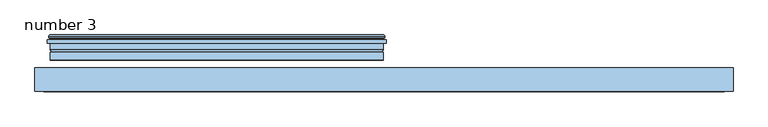
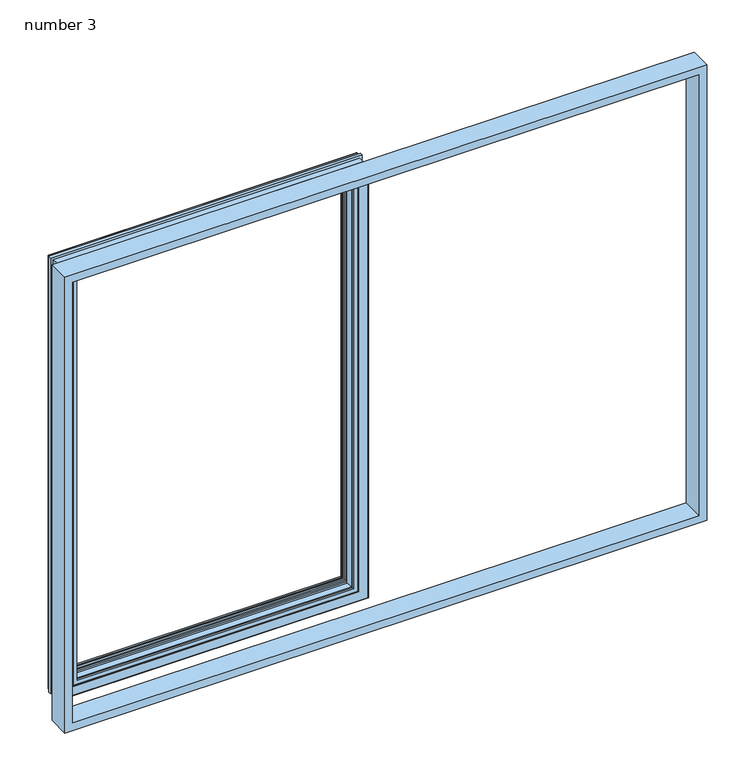
"""IFC4 building model written with IfcOpenShell, lengths in millimetres: window geometry, Window-Exterior-Sierra-Horizontal_Sliding_XO-36inch_Width-Standard : number 3."""

from ifc_helpers import new_model, si_unit, frame, origin, place, context, project, spatial, polyline, ellipse_curve, outline, extrude, source, transform, mapped, element, save
from ifc_brep_helpers import plane_surface, cylinder_surface, revolved_surface, advanced_brep


def number_3_e313addd(model_context):
    return source(origin(), model_context, "Body", "SolidModel", [
        advanced_brep(
        [(-554.92015, 35.099625, 967.49235), (-554.92015, 33.9637671, 967.49235), (-29.27985, 33.9637671, 967.49235), (-29.27985, 35.099625, 967.49235), (-553.0833265, 37.5426644, 969.3291735), (-552.8937762, 35.099625, 969.5187238), (-31.3062238, 35.099625, 969.5187238), (-31.1166735, 37.5426644, 969.3291735), (-560.88915, 40.078025, 961.52335), (-23.31085, 40.078025, 961.52335), (-560.88915, 42.465625, 961.52335), (-23.31085, 42.465625, 961.52335), (-585.57795, 40.078025, 936.83455), (-583.19035, 42.465625, 939.22215), (-1.00965, 42.465625, 939.22215), (1.37795, 40.078025, 936.83455), (-585.57795, 37.512625, 936.83455), (1.37795, 37.512625, 936.83455), (-583.54595, 35.836225, 938.86655), (-583.54595, 37.512625, 938.86655), (-0.65405, 37.512625, 938.86655), (-0.65405, 35.836225, 938.86655), (-580.24395, 33.931225, 942.16855), (-580.24395, 35.836225, 942.16855), (-3.95605, 35.836225, 942.16855), (-3.95605, 33.931225, 942.16855), (-588.16875, 28.317825, 934.24375), (-588.16875, 33.931225, 934.24375), (3.96875, 33.931225, 934.24375), (3.96875, 28.317825, 934.24375), (-582.86015, 16.125825, 939.55235), (-582.86015, 28.317825, 939.55235), (-1.33985, 28.317825, 939.55235), (-1.33985, 16.125825, 939.55235), (-582.86015, 12.163425, 939.55235), (-1.33985, 12.163425, 939.55235), (-582.86015, -1.171575, 939.55235), (-1.33985, -1.171575, 939.55235), (-582.04735, -1.984375, 940.36515), (-2.15265, -1.984375, 940.36515), (-563.75935, -0.103857, 958.65315), (-563.75935, -1.984375, 958.65315), (-20.44065, -1.984375, 958.65315), (-20.44065, -0.103857, 958.65315), (-562.1584612, -1.704057, 960.2540388), (-562.1584612, -0.103857, 960.2540388), (-22.0415388, -0.103857, 960.2540388), (-22.0415388, -1.704057, 960.2540388), (-554.6146612, 2.0638625, 967.7978388), (-554.6146612, -1.704057, 967.7978388), (-29.5853388, -1.704057, 967.7978388), (-29.5853388, 2.0638625, 967.7978388), (-551.4396612, 13.891543, 970.9728388), (-552.4523112, 2.0638625, 969.9601888), (-31.7476888, 2.0638625, 969.9601888), (-32.7603388, 13.891543, 970.9728388), (-563.75935, 11.5032541, 958.65315), (-561.3710612, 13.891543, 961.0414388), (-22.8289388, 13.891543, 961.0414388), (-20.44065, 11.5032541, 958.65315), (-563.75935, 32.940625, 958.65315), (-20.44065, 32.940625, 958.65315), (-559.1555891, 33.9637671, 963.2569109), (-560.1787312, 32.940625, 962.2337688), (-24.0212688, 32.940625, 962.2337688), (-25.0444109, 33.9637671, 963.2569109), (-29.27985, 33.9637671, 1775.70765), (-29.27985, 35.099625, 1775.70765), (-31.3062238, 35.099625, 1773.6812762), (-31.1166735, 37.5426644, 1773.8708265), (-23.31085, 40.078025, 1781.67665), (-23.31085, 42.465625, 1781.67665), (-1.00965, 42.465625, 1803.97785), (1.37795, 40.078025, 1806.36545), (1.37795, 37.512625, 1806.36545), (-0.65405, 37.512625, 1804.33345), (-0.65405, 35.836225, 1804.33345), (-3.95605, 35.836225, 1801.03145), (-3.95605, 33.931225, 1801.03145), (3.96875, 33.931225, 1808.95625), (3.96875, 28.317825, 1808.95625), (-1.33985, 28.317825, 1803.64765), (-1.33985, 16.125825, 1803.64765), (-1.33985, 12.163425, 1803.64765), (-1.33985, -1.171575, 1803.64765), (-2.15265, -1.984375, 1802.83485), (-20.44065, -1.984375, 1784.54685), (-20.44065, -0.103857, 1784.54685), (-22.0415388, -0.103857, 1782.9459612), (-22.0415388, -1.704057, 1782.9459612), (-29.5853388, -1.704057, 1775.4021612), (-29.5853388, 2.0638625, 1775.4021612), (-31.7476888, 2.0638625, 1773.2398112), (-32.7603388, 13.891543, 1772.2271612), (-22.8289388, 13.891543, 1782.1585612), (-20.44065, 11.5032541, 1784.54685), (-20.44065, 32.940625, 1784.54685), (-24.0212688, 32.940625, 1780.9662312), (-25.0444109, 33.9637671, 1779.9430891), (-554.92015, 33.9637671, 1775.70765), (-554.92015, 35.099625, 1775.70765), (-552.8937762, 35.099625, 1773.6812762), (-553.0833265, 37.5426644, 1773.8708265), (-560.88915, 40.078025, 1781.67665), (-560.88915, 42.465625, 1781.67665), (-583.19035, 42.465625, 1803.97785), (-585.57795, 40.078025, 1806.36545), (-585.57795, 37.512625, 1806.36545), (-583.54595, 37.512625, 1804.33345), (-583.54595, 35.836225, 1804.33345), (-580.24395, 35.836225, 1801.03145), (-580.24395, 33.931225, 1801.03145), (-588.16875, 33.931225, 1808.95625), (-588.16875, 28.317825, 1808.95625), (-582.86015, 28.317825, 1803.64765), (-582.86015, 16.125825, 1803.64765), (-582.86015, 12.163425, 1803.64765), (-582.86015, -1.171575, 1803.64765), (-582.04735, -1.984375, 1802.83485), (-563.75935, -1.984375, 1784.54685), (-563.75935, -0.103857, 1784.54685), (-562.1584612, -0.103857, 1782.9459612), (-562.1584612, -1.704057, 1782.9459612), (-554.6146612, -1.704057, 1775.4021612), (-554.6146612, 2.0638625, 1775.4021612), (-552.4523112, 2.0638625, 1773.2398112), (-551.4396612, 13.891543, 1772.2271612), (-561.3710612, 13.891543, 1782.1585612), (-563.75935, 11.5032541, 1784.54685), (-563.75935, 32.940625, 1784.54685), (-560.1787312, 32.940625, 1780.9662312), (-559.1555891, 33.9637671, 1779.9430891)],
        [
            (0, 1),
            (1, 2),
            (2, 3),
            (3, 0),
            (4, 5),
            (5, 6),
            (6, 7),
            (7, 4),
            (8, 4),
            (7, 9),
            (9, 8),
            (10, 8),
            (9, 11),
            (11, 10),
            (12, 13, ellipse_curve(frame((-583.19035, 40.078025, 939.22215), z_axis=(0.7071067811865475, 0.0, -0.7071067811865475), x_axis=(-0.7071067811865476, 0.0, -0.7071067811865474)), 3.3765763, 2.3876)),
            (13, 14),
            (14, 15, ellipse_curve(frame((-1.00965, 40.078025, 939.22215), z_axis=(-0.7071067811865475, 0.0, -0.7071067811865475), x_axis=(-0.7071067811865476, 0.0, 0.7071067811865474)), 3.3765763, 2.3876)),
            (15, 12),
            (16, 12),
            (15, 17),
            (17, 16),
            (18, 19),
            (19, 20),
            (20, 21),
            (21, 18),
            (22, 23),
            (23, 24),
            (24, 25),
            (25, 22),
            (26, 27),
            (27, 28),
            (28, 29),
            (29, 26),
            (30, 31),
            (31, 32),
            (32, 33),
            (33, 30),
            (34, 30, ellipse_curve(frame((-582.86015, 14.144625, 939.55235), z_axis=(-0.7071067811865475, 0.0, 0.7071067811865475), x_axis=(0.7071067811865476, 0.0, 0.7071067811865474)), 2.8018399, 1.9812)),
            (33, 35, ellipse_curve(frame((-1.33985, 14.144625, 939.55235), z_axis=(0.7071067811865475, 0.0, 0.7071067811865475), x_axis=(0.7071067811865476, 0.0, -0.7071067811865474)), 2.8018399, 1.9812)),
            (35, 34),
            (36, 34),
            (35, 37),
            (37, 36),
            (38, 36, ellipse_curve(frame((-582.04735, -1.171575, 940.36515), z_axis=(0.7071067811865475, 0.0, -0.7071067811865475), x_axis=(-0.7071067811865476, 0.0, -0.7071067811865474)), 1.1494728, 0.8128)),
            (37, 39, ellipse_curve(frame((-2.15265, -1.171575, 940.36515), z_axis=(-0.7071067811865475, 0.0, -0.7071067811865475), x_axis=(-0.7071067811865476, 0.0, 0.7071067811865474)), 1.1494728, 0.8128)),
            (39, 38),
            (40, 41),
            (41, 42),
            (42, 43),
            (43, 40),
            (44, 45),
            (45, 46),
            (46, 47),
            (47, 44),
            (48, 49),
            (49, 50),
            (50, 51),
            (51, 48),
            (52, 53),
            (53, 54),
            (54, 55),
            (55, 52),
            (56, 57),
            (57, 58),
            (58, 59),
            (59, 56),
            (60, 56),
            (59, 61),
            (61, 60),
            (62, 63),
            (63, 64),
            (64, 65),
            (65, 62),
            (2, 66),
            (66, 67),
            (67, 3),
            (6, 68),
            (68, 69),
            (69, 7),
            (69, 70),
            (70, 9),
            (70, 71),
            (71, 11),
            (14, 72),
            (72, 73, ellipse_curve(frame((-1.00965, 40.078025, 1803.97785), z_axis=(0.7071067811865475, 0.0, -0.7071067811865475), x_axis=(-0.7071067811865474, 0.0, -0.7071067811865476)), 3.3765763, 2.3876)),
            (73, 15),
            (73, 74),
            (74, 17),
            (20, 75),
            (75, 76),
            (76, 21),
            (24, 77),
            (77, 78),
            (78, 25),
            (28, 79),
            (79, 80),
            (80, 29),
            (32, 81),
            (81, 82),
            (82, 33),
            (82, 83, ellipse_curve(frame((-1.33985, 14.144625, 1803.64765), z_axis=(-0.7071067811865475, 0.0, 0.7071067811865475), x_axis=(0.7071067811865474, 0.0, 0.7071067811865476)), 2.8018399, 1.9812)),
            (83, 35),
            (83, 84),
            (84, 37),
            (84, 85, ellipse_curve(frame((-2.15265, -1.171575, 1802.83485), z_axis=(0.7071067811865475, 0.0, -0.7071067811865475), x_axis=(-0.7071067811865474, 0.0, -0.7071067811865476)), 1.1494728, 0.8128)),
            (85, 39),
            (42, 86),
            (86, 87),
            (87, 43),
            (46, 88),
            (88, 89),
            (89, 47),
            (50, 90),
            (90, 91),
            (91, 51),
            (54, 92),
            (92, 93),
            (93, 55),
            (58, 94),
            (94, 95),
            (95, 59),
            (95, 96),
            (96, 61),
            (64, 97),
            (97, 98),
            (98, 65),
            (66, 99),
            (99, 100),
            (100, 67),
            (68, 101),
            (101, 102),
            (102, 69),
            (102, 103),
            (103, 70),
            (103, 104),
            (104, 71),
            (72, 105),
            (105, 106, ellipse_curve(frame((-583.19035, 40.078025, 1803.97785), z_axis=(0.7071067811865475, 0.0, 0.7071067811865475), x_axis=(0.7071067811865476, 0.0, -0.7071067811865474)), 3.3765763, 2.3876)),
            (106, 73),
            (106, 107),
            (107, 74),
            (75, 108),
            (108, 109),
            (109, 76),
            (77, 110),
            (110, 111),
            (111, 78),
            (79, 112),
            (112, 113),
            (113, 80),
            (81, 114),
            (114, 115),
            (115, 82),
            (115, 116, ellipse_curve(frame((-582.86015, 14.144625, 1803.64765), z_axis=(-0.7071067811865475, 0.0, -0.7071067811865475), x_axis=(-0.7071067811865476, 0.0, 0.7071067811865474)), 2.8018399, 1.9812)),
            (116, 83),
            (116, 117),
            (117, 84),
            (117, 118, ellipse_curve(frame((-582.04735, -1.171575, 1802.83485), z_axis=(0.7071067811865475, 0.0, 0.7071067811865475), x_axis=(0.7071067811865476, 0.0, -0.7071067811865474)), 1.1494728, 0.8128)),
            (118, 85),
            (86, 119),
            (119, 120),
            (120, 87),
            (88, 121),
            (121, 122),
            (122, 89),
            (90, 123),
            (123, 124),
            (124, 91),
            (92, 125),
            (125, 126),
            (126, 93),
            (94, 127),
            (127, 128),
            (128, 95),
            (128, 129),
            (129, 96),
            (97, 130),
            (130, 131),
            (131, 98),
            (131, 62),
            (1, 99),
            (0, 100),
            (5, 101),
            (4, 102),
            (8, 103),
            (10, 104),
            (13, 105),
            (12, 106),
            (16, 107),
            (19, 108),
            (18, 109),
            (23, 110),
            (22, 111),
            (27, 112),
            (26, 113),
            (31, 114),
            (30, 115),
            (34, 116),
            (36, 117),
            (38, 118),
            (41, 119),
            (40, 120),
            (45, 121),
            (44, 122),
            (49, 123),
            (48, 124),
            (53, 125),
            (52, 126),
            (57, 127),
            (56, 128),
            (60, 129),
            (63, 130),
        ],
        [
            plane_surface(frame((-554.92015, 33.9637671, 967.49235), z_axis=(0.0, 0.0, 1.0), x_axis=(1.0, 0.0, 0.0))),
            plane_surface(frame((-552.8937762, 35.099625, 969.5187238), z_axis=(0.0, 0.07735544009934271, 0.9970035786731345), x_axis=(1.0, 0.0, 0.0))),
            plane_surface(frame((-553.0833265, 37.5426644, 969.3291735), z_axis=(0.0, 0.9510889261909004, 0.3089172291683326), x_axis=(1.0, 0.0, 0.0))),
            plane_surface(frame((-560.88915, 40.078025, 961.52335), z_axis=(0.0, 0.0, 1.0), x_axis=(1.0, 0.0, 0.0))),
            cylinder_surface(frame((-588.16875, 40.078025, 939.22215), z_axis=(-1.0, 0.0, 0.0), x_axis=(0.0, -1.0, 0.0)), 2.3876),
            plane_surface(frame((-585.57795, 40.078025, 936.83455), z_axis=(0.0, 0.0, -1.0), x_axis=(1.0, 0.0, 0.0))),
            plane_surface(frame((-583.54595, 37.512625, 938.86655), z_axis=(0.0, 0.0, -1.0), x_axis=(1.0, 0.0, 0.0))),
            plane_surface(frame((-580.24395, 35.836225, 942.16855), z_axis=(0.0, 0.0, -1.0), x_axis=(1.0, 0.0, 0.0))),
            plane_surface(frame((-588.16875, 33.931225, 934.24375), z_axis=(0.0, 0.0, -1.0), x_axis=(1.0, 0.0, 0.0))),
            plane_surface(frame((-582.86015, 28.317825, 939.55235), z_axis=(0.0, 0.0, -1.0), x_axis=(1.0, 0.0, 0.0))),
            revolved_surface(polyline([(0.6413499930890794, 12.163425, 939.55235), (-584.841349993089, 12.163425, 939.55235)]), (-588.16875, 14.144625, 939.55235), (1.0, 0.0, 0.0)),
            plane_surface(frame((-582.86015, 12.163425, 939.55235), z_axis=(0.0, 0.0, -1.0), x_axis=(1.0, 0.0, 0.0))),
            cylinder_surface(frame((-588.16875, -1.171575, 940.36515), z_axis=(-1.0, 0.0, 0.0), x_axis=(0.0, -1.0, 0.0)), 0.8128),
            plane_surface(frame((-563.75935, -1.984375, 958.65315), z_axis=(0.0, 0.0, 1.0), x_axis=(1.0, 0.0, 0.0))),
            plane_surface(frame((-562.1584612, -0.103857, 960.2540388), z_axis=(0.0, 0.0, -1.0), x_axis=(1.0, 0.0, 0.0))),
            plane_surface(frame((-554.6146612, -1.704057, 967.7978388), z_axis=(0.0, 0.0, 1.0), x_axis=(1.0, 0.0, 0.0))),
            plane_surface(frame((-552.4523112, 2.0638625, 969.9601888), z_axis=(0.0, -0.08530487454184647, 0.996354895797376), x_axis=(1.0, 0.0, 0.0))),
            plane_surface(frame((-561.3710612, 13.891543, 961.0414388), z_axis=(0.0, 0.7071067811865713, -0.7071067811865238), x_axis=(1.0, 0.0, 0.0))),
            plane_surface(frame((-563.75935, 11.5032541, 958.65315), z_axis=(0.0, 0.0, 1.0), x_axis=(1.0, 0.0, 0.0))),
            plane_surface(frame((-560.1787312, 32.940625, 962.2337688), z_axis=(0.0, -0.7071067811861558, 0.7071067811869393), x_axis=(1.0, 0.0, 0.0))),
            plane_surface(frame((-29.27985, 33.9637671, 967.49235), z_axis=(-1.0, 0.0, 0.0), x_axis=(0.0, 0.0, 1.0))),
            plane_surface(frame((-31.3062238, 35.099625, 969.5187238), z_axis=(-0.9970035786731345, 0.07735544009934266, 0.0), x_axis=(0.0, 0.0, 1.0))),
            plane_surface(frame((-31.1166735, 37.5426644, 969.3291735), z_axis=(-0.30891722916833264, 0.9510889261909004, 0.0), x_axis=(0.0, 0.0, 1.0))),
            plane_surface(frame((-23.31085, 40.078025, 961.52335), z_axis=(-1.0, 0.0, 0.0), x_axis=(0.0, 0.0, 1.0))),
            cylinder_surface(frame((-1.00965, 40.078025, 934.24375), z_axis=(0.0, 0.0, -1.0), x_axis=(0.0, -1.0, 0.0)), 2.3876),
            plane_surface(frame((1.37795, 40.078025, 936.83455), z_axis=(1.0, 0.0, 0.0), x_axis=(0.0, 0.0, 1.0))),
            plane_surface(frame((-0.65405, 37.512625, 938.86655), z_axis=(1.0, 0.0, 0.0), x_axis=(0.0, 0.0, 1.0))),
            plane_surface(frame((-3.95605, 35.836225, 942.16855), z_axis=(1.0, 0.0, 0.0), x_axis=(0.0, 0.0, 1.0))),
            plane_surface(frame((3.96875, 33.931225, 934.24375), z_axis=(1.0, 0.0, 0.0), x_axis=(0.0, 0.0, 1.0))),
            plane_surface(frame((-1.33985, 28.317825, 939.55235), z_axis=(1.0, 0.0, 0.0), x_axis=(0.0, 0.0, 1.0))),
            revolved_surface(polyline([(-1.33985, 12.163425, 1805.6288499930893), (-1.33985, 12.163425, 937.571150006911)]), (-1.33985, 14.144625, 934.24375), (0.0, 0.0, 1.0)),
            plane_surface(frame((-1.33985, 12.163425, 939.55235), z_axis=(1.0, 0.0, 0.0), x_axis=(0.0, 0.0, 1.0))),
            cylinder_surface(frame((-2.15265, -1.171575, 934.24375), z_axis=(0.0, 0.0, -1.0), x_axis=(0.0, -1.0, 0.0)), 0.8128),
            plane_surface(frame((-20.44065, -1.984375, 958.65315), z_axis=(-1.0, 0.0, 0.0), x_axis=(0.0, 0.0, 1.0))),
            plane_surface(frame((-22.0415388, -0.103857, 960.2540388), z_axis=(1.0, 0.0, 0.0), x_axis=(0.0, 0.0, 1.0))),
            plane_surface(frame((-29.5853388, -1.704057, 967.7978388), z_axis=(-1.0, 0.0, 0.0), x_axis=(0.0, 0.0, 1.0))),
            plane_surface(frame((-31.7476888, 2.0638625, 969.9601888), z_axis=(-0.996354895797376, -0.08530487454184653, 0.0), x_axis=(0.0, 0.0, 1.0))),
            plane_surface(frame((-22.8289388, 13.891543, 961.0414388), z_axis=(0.7071067811865238, 0.7071067811865713, 0.0), x_axis=(0.0, 0.0, 1.0))),
            plane_surface(frame((-20.44065, 11.5032541, 958.65315), z_axis=(-1.0, 0.0, 0.0), x_axis=(0.0, 0.0, 1.0))),
            plane_surface(frame((-24.0212688, 32.940625, 962.2337688), z_axis=(-0.7071067811869393, -0.7071067811861558, 0.0), x_axis=(0.0, 0.0, 1.0))),
            plane_surface(frame((-29.27985, 33.9637671, 1775.70765), z_axis=(0.0, 0.0, -1.0), x_axis=(-1.0, 0.0, 0.0))),
            plane_surface(frame((-31.3062238, 35.099625, 1773.6812762), z_axis=(0.0, 0.0773554400993426, -0.9970035786731345), x_axis=(-1.0, 0.0, 0.0))),
            plane_surface(frame((-31.1166735, 37.5426644, 1773.8708265), z_axis=(0.0, 0.9510889261909004, -0.3089172291683327), x_axis=(-1.0, 0.0, 0.0))),
            plane_surface(frame((-23.31085, 40.078025, 1781.67665), z_axis=(0.0, 0.0, -1.0), x_axis=(-1.0, 0.0, 0.0))),
            cylinder_surface(frame((3.96875, 40.078025, 1803.97785), z_axis=(1.0, 0.0, 0.0), x_axis=(0.0, -1.0, 0.0)), 2.3876),
            plane_surface(frame((1.37795, 40.078025, 1806.36545), z_axis=(0.0, 0.0, 1.0), x_axis=(-1.0, 0.0, 0.0))),
            plane_surface(frame((-0.65405, 37.512625, 1804.33345), z_axis=(0.0, 0.0, 1.0), x_axis=(-1.0, 0.0, 0.0))),
            plane_surface(frame((-3.95605, 35.836225, 1801.03145), z_axis=(0.0, 0.0, 1.0), x_axis=(-1.0, 0.0, 0.0))),
            plane_surface(frame((3.96875, 33.931225, 1808.95625), z_axis=(0.0, 0.0, 1.0), x_axis=(-1.0, 0.0, 0.0))),
            plane_surface(frame((-1.33985, 28.317825, 1803.64765), z_axis=(0.0, 0.0, 1.0), x_axis=(-1.0, 0.0, 0.0))),
            revolved_surface(polyline([(-584.841349993089, 12.163425, 1803.64765), (0.6413499930890376, 12.163425, 1803.64765)]), (3.96875, 14.144625, 1803.64765), (-1.0, 0.0, 0.0)),
            plane_surface(frame((-1.33985, 12.163425, 1803.64765), z_axis=(0.0, 0.0, 1.0), x_axis=(-1.0, 0.0, 0.0))),
            cylinder_surface(frame((3.96875, -1.171575, 1802.83485), z_axis=(1.0, 0.0, 0.0), x_axis=(0.0, -1.0, 0.0)), 0.8128),
            plane_surface(frame((-20.44065, -1.984375, 1784.54685), z_axis=(0.0, 0.0, -1.0), x_axis=(-1.0, 0.0, 0.0))),
            plane_surface(frame((-22.0415388, -0.103857, 1782.9459612), z_axis=(0.0, 0.0, 1.0), x_axis=(-1.0, 0.0, 0.0))),
            plane_surface(frame((-29.5853388, -1.704057, 1775.4021612), z_axis=(0.0, 0.0, -1.0), x_axis=(-1.0, 0.0, 0.0))),
            plane_surface(frame((-31.7476888, 2.0638625, 1773.2398112), z_axis=(0.0, -0.08530487454184658, -0.996354895797376), x_axis=(-1.0, 0.0, 0.0))),
            plane_surface(frame((-22.8289388, 13.891543, 1782.1585612), z_axis=(0.0, 0.7071067811865713, 0.7071067811865238), x_axis=(-1.0, 0.0, 0.0))),
            plane_surface(frame((-20.44065, 11.5032541, 1784.54685), z_axis=(0.0, 0.0, -1.0), x_axis=(-1.0, 0.0, 0.0))),
            plane_surface(frame((-24.0212688, 32.940625, 1780.9662312), z_axis=(0.0, -0.7071067811861558, -0.7071067811869393), x_axis=(-1.0, 0.0, 0.0))),
            plane_surface(frame((-559.1555891, 33.9637671, 1779.9430891), z_axis=(0.0, -1.0, 0.0), x_axis=(0.0, 0.0, -1.0))),
            plane_surface(frame((-554.92015, 33.9637671, 1775.70765), z_axis=(1.0, 0.0, 0.0), x_axis=(0.0, 0.0, -1.0))),
            plane_surface(frame((-554.92015, 35.099625, 1775.70765), z_axis=(0.0, -1.0, 0.0), x_axis=(0.0, 0.0, -1.0))),
            plane_surface(frame((-552.8937762, 35.099625, 1773.6812762), z_axis=(0.9970035786731345, 0.07735544009934266, 0.0), x_axis=(0.0, 0.0, -1.0))),
            plane_surface(frame((-553.0833265, 37.5426644, 1773.8708265), z_axis=(0.30891722916833264, 0.9510889261909004, 0.0), x_axis=(0.0, 0.0, -1.0))),
            plane_surface(frame((-560.88915, 40.078025, 1781.67665), z_axis=(1.0, 0.0, 0.0), x_axis=(0.0, 0.0, -1.0))),
            plane_surface(frame((-560.88915, 42.465625, 1781.67665), z_axis=(0.0, 1.0, 0.0), x_axis=(0.0, 0.0, -1.0))),
            cylinder_surface(frame((-583.19035, 40.078025, 1808.95625), z_axis=(0.0, 0.0, 1.0), x_axis=(0.0, -1.0, 0.0)), 2.3876),
            plane_surface(frame((-585.57795, 40.078025, 1806.36545), z_axis=(-1.0, 0.0, 0.0), x_axis=(0.0, 0.0, -1.0))),
            plane_surface(frame((-585.57795, 37.512625, 1806.36545), z_axis=(0.0, -1.0, 0.0), x_axis=(0.0, 0.0, -1.0))),
            plane_surface(frame((-583.54595, 37.512625, 1804.33345), z_axis=(-1.0, 0.0, 0.0), x_axis=(0.0, 0.0, -1.0))),
            plane_surface(frame((-583.54595, 35.836225, 1804.33345), z_axis=(0.0, -1.0, 0.0), x_axis=(0.0, 0.0, -1.0))),
            plane_surface(frame((-580.24395, 35.836225, 1801.03145), z_axis=(-1.0, 0.0, 0.0), x_axis=(0.0, 0.0, -1.0))),
            plane_surface(frame((-580.24395, 33.931225, 1801.03145), z_axis=(0.0, 1.0, 0.0), x_axis=(0.0, 0.0, -1.0))),
            plane_surface(frame((-588.16875, 33.931225, 1808.95625), z_axis=(-1.0, 0.0, 0.0), x_axis=(0.0, 0.0, -1.0))),
            plane_surface(frame((-588.16875, 28.317825, 1808.95625), z_axis=(0.0, -1.0, 0.0), x_axis=(0.0, 0.0, -1.0))),
            plane_surface(frame((-582.86015, 28.317825, 1803.64765), z_axis=(-1.0, 0.0, 0.0), x_axis=(0.0, 0.0, -1.0))),
            revolved_surface(polyline([(-582.86015, 12.163425, 937.571150006911), (-582.86015, 12.163425, 1805.6288499930893)]), (-582.86015, 14.144625, 1808.95625), (0.0, 0.0, -1.0)),
            plane_surface(frame((-582.86015, 12.163425, 1803.64765), z_axis=(-1.0, 0.0, 0.0), x_axis=(0.0, 0.0, -1.0))),
            cylinder_surface(frame((-582.04735, -1.171575, 1808.95625), z_axis=(0.0, 0.0, 1.0), x_axis=(0.0, -1.0, 0.0)), 0.8128),
            plane_surface(frame((-582.04735, -1.984375, 1802.83485), z_axis=(0.0, -1.0, 0.0), x_axis=(0.0, 0.0, -1.0))),
            plane_surface(frame((-563.75935, -1.984375, 1784.54685), z_axis=(1.0, 0.0, 0.0), x_axis=(0.0, 0.0, -1.0))),
            plane_surface(frame((-563.75935, -0.103857, 1784.54685), z_axis=(0.0, -1.0, 0.0), x_axis=(0.0, 0.0, -1.0))),
            plane_surface(frame((-562.1584612, -0.103857, 1782.9459612), z_axis=(-1.0, 0.0, 0.0), x_axis=(0.0, 0.0, -1.0))),
            plane_surface(frame((-562.1584612, -1.704057, 1782.9459612), z_axis=(0.0, -1.0, 0.0), x_axis=(0.0, 0.0, -1.0))),
            plane_surface(frame((-554.6146612, -1.704057, 1775.4021612), z_axis=(1.0, 0.0, 0.0), x_axis=(0.0, 0.0, -1.0))),
            plane_surface(frame((-554.6146612, 2.0638625, 1775.4021612), z_axis=(0.0, -1.0, 0.0), x_axis=(0.0, 0.0, -1.0))),
            plane_surface(frame((-552.4523112, 2.0638625, 1773.2398112), z_axis=(0.996354895797376, -0.08530487454184653, 0.0), x_axis=(0.0, 0.0, -1.0))),
            plane_surface(frame((-551.4396612, 13.891543, 1772.2271612), z_axis=(0.0, 1.0, 0.0), x_axis=(0.0, 0.0, -1.0))),
            plane_surface(frame((-561.3710612, 13.891543, 1782.1585612), z_axis=(-0.7071067811865238, 0.7071067811865713, 0.0), x_axis=(0.0, 0.0, -1.0))),
            plane_surface(frame((-563.75935, 11.5032541, 1784.54685), z_axis=(1.0, 0.0, 0.0), x_axis=(0.0, 0.0, -1.0))),
            plane_surface(frame((-563.75935, 32.940625, 1784.54685), z_axis=(0.0, -1.0, 0.0), x_axis=(0.0, 0.0, -1.0))),
            plane_surface(frame((-560.1787312, 32.940625, 1780.9662312), z_axis=(0.7071067811869393, -0.7071067811861558, 0.0), x_axis=(0.0, 0.0, -1.0))),
        ],
        [
            (0, [[1, 2, 3, 4]]),
            (1, [[5, 6, 7, 8]]),
            (2, [[9, -8, 10, 11]]),
            (3, [[12, -11, 13, 14]]),
            (4, [[15, 16, 17, 18]]),
            (5, [[19, -18, 20, 21]]),
            (6, [[22, 23, 24, 25]]),
            (7, [[26, 27, 28, 29]]),
            (8, [[30, 31, 32, 33]]),
            (9, [[34, 35, 36, 37]]),
            (10, [[38, -37, 39, 40]]),
            (11, [[41, -40, 42, 43]]),
            (12, [[44, -43, 45, 46]]),
            (13, [[47, 48, 49, 50]]),
            (14, [[51, 52, 53, 54]]),
            (15, [[55, 56, 57, 58]]),
            (16, [[59, 60, 61, 62]]),
            (17, [[63, 64, 65, 66]]),
            (18, [[67, -66, 68, 69]]),
            (19, [[70, 71, 72, 73]]),
            (20, [[-3, 74, 75, 76]]),
            (21, [[-7, 77, 78, 79]]),
            (22, [[-10, -79, 80, 81]]),
            (23, [[-13, -81, 82, 83]]),
            (24, [[-17, 84, 85, 86]]),
            (25, [[-20, -86, 87, 88]]),
            (26, [[-24, 89, 90, 91]]),
            (27, [[-28, 92, 93, 94]]),
            (28, [[-32, 95, 96, 97]]),
            (29, [[-36, 98, 99, 100]]),
            (30, [[-39, -100, 101, 102]]),
            (31, [[-42, -102, 103, 104]]),
            (32, [[-45, -104, 105, 106]]),
            (33, [[-49, 107, 108, 109]]),
            (34, [[-53, 110, 111, 112]]),
            (35, [[-57, 113, 114, 115]]),
            (36, [[-61, 116, 117, 118]]),
            (37, [[-65, 119, 120, 121]]),
            (38, [[-68, -121, 122, 123]]),
            (39, [[-72, 124, 125, 126]]),
            (40, [[-75, 127, 128, 129]]),
            (41, [[-78, 130, 131, 132]]),
            (42, [[-80, -132, 133, 134]]),
            (43, [[-82, -134, 135, 136]]),
            (44, [[-85, 137, 138, 139]]),
            (45, [[-87, -139, 140, 141]]),
            (46, [[-90, 142, 143, 144]]),
            (47, [[-93, 145, 146, 147]]),
            (48, [[-96, 148, 149, 150]]),
            (49, [[-99, 151, 152, 153]]),
            (50, [[-101, -153, 154, 155]]),
            (51, [[-103, -155, 156, 157]]),
            (52, [[-105, -157, 158, 159]]),
            (53, [[-108, 160, 161, 162]]),
            (54, [[-111, 163, 164, 165]]),
            (55, [[-114, 166, 167, 168]]),
            (56, [[-117, 169, 170, 171]]),
            (57, [[-120, 172, 173, 174]]),
            (58, [[-122, -174, 175, 176]]),
            (59, [[-125, 177, 178, 179]]),
            (60, [[-126, -179, 180, -73], [181, -127, -74, -2]]),
            (61, [[-128, -181, -1, 182]]),
            (62, [[-76, -129, -182, -4], [183, -130, -77, -6]]),
            (63, [[-131, -183, -5, 184]]),
            (64, [[-133, -184, -9, 185]]),
            (65, [[-135, -185, -12, 186]]),
            (66, [[187, -137, -84, -16], [-83, -136, -186, -14]]),
            (67, [[-138, -187, -15, 188]]),
            (68, [[-140, -188, -19, 189]]),
            (69, [[-88, -141, -189, -21], [190, -142, -89, -23]]),
            (70, [[-143, -190, -22, 191]]),
            (71, [[-91, -144, -191, -25], [192, -145, -92, -27]]),
            (72, [[-146, -192, -26, 193]]),
            (73, [[194, -148, -95, -31], [-94, -147, -193, -29]]),
            (74, [[-149, -194, -30, 195]]),
            (75, [[-97, -150, -195, -33], [196, -151, -98, -35]]),
            (76, [[-152, -196, -34, 197]]),
            (77, [[-154, -197, -38, 198]]),
            (78, [[-156, -198, -41, 199]]),
            (79, [[-158, -199, -44, 200]]),
            (80, [[-106, -159, -200, -46], [201, -160, -107, -48]]),
            (81, [[-161, -201, -47, 202]]),
            (82, [[-109, -162, -202, -50], [203, -163, -110, -52]]),
            (83, [[-164, -203, -51, 204]]),
            (84, [[-112, -165, -204, -54], [205, -166, -113, -56]]),
            (85, [[-167, -205, -55, 206]]),
            (86, [[-115, -168, -206, -58], [207, -169, -116, -60]]),
            (87, [[-170, -207, -59, 208]]),
            (88, [[209, -172, -119, -64], [-118, -171, -208, -62]]),
            (89, [[-173, -209, -63, 210]]),
            (90, [[-175, -210, -67, 211]]),
            (91, [[-123, -176, -211, -69], [212, -177, -124, -71]]),
            (92, [[-178, -212, -70, -180]]),
        ],
    ),
        extrude(outline(polyline([(1828.8, 609.6), (1828.8, -609.6), (914.4, -609.6), (914.4, 609.6), (1828.8, 609.6)]), holes=[polyline([(929.4367932, 594.5632068), (929.4367932, -594.5632068), (1813.7632068, -594.5632068), (1813.7632068, 594.5632068), (929.4367932, 594.5632068)])]), frame((0.0, -56.35625, 0.0), z_axis=(0.0, 1.0, 0.0), x_axis=(0.0, 0.0, 1.0)), (0.0, 0.0, 1.0), 41.7512996),
    ])


if __name__ == "__main__":
    model = new_model("IFC4")
    model_context = context("Model", 3, world=origin())
    ifc_project = project(units=[si_unit("LENGTHUNIT", "METRE", prefix="MILLI")], contexts=[model_context])
    site = spatial("IfcSite", under=ifc_project)
    building = spatial("IfcBuilding", under=site)
    placement = place(None, origin())
    number_3_shape = number_3_e313addd(model_context)
    element("IfcWindow", 1, ObjectType="Window-Exterior-Sierra-Horizontal_Sliding_XO-36inch_Width-Standard : number 3", at=placement, inside=building, context=model_context, shape_type="MappedRepresentation", body=[
        mapped(number_3_shape, transform((0.0, 0.0, 0.0), x_axis=(1.0, 0.0, 0.0), y_axis=(0.0, 1.0, 0.0), z_axis=(0.0, 0.0, 1.0))),
    ])
    save(model, "model.ifc")

# Revit data of these elements
# Type "Window-Exterior-Sierra-Horizontal_Sliding_XO-36inch_Width-Standard : number 3"
#   Type Mark = "51"
#   URL = "http://www.sierrapacificwindows.com"
#   Triple Glaze Note = "Triple glazed options with respective limits"
#   Simulite Note = "Custom Simulite Options Available"
#   Product data url = "https://bimobject.com/sierrapacificwindows/product/sierrapacificwindows_horizontal-sliding-windows"
#   Product Page URL = "http://www.sierrapacificwindows.com/horizontal-sliding-windows.cfm"
#   Product Documentation Link = "http://www.sierrapacificwindows.com/architectural/drawings/pdfs/c-ws_13.pdf"
#   Model = "C-WS-3648"
#   Manufacturer = "Sierra Pacific Windows"
#   Jamb Extension Note = "Extension Jamb may be applied on some applications. Contact your SPW sales rep. for more information"
#   Glass Type = "Insulated Glass"
#   Description = "Energy efficient, durable, and secure window"
#   Construction Type = "Wood/Clad"
#   Assembly Code = "B2030230"
#   Window Pane Thickness = 0' - 0 3/4"
#   Vertical Simulite Length = 2' - 9"
#   Thickness = 0' - 1 3/4"
#   Simulite Wood Thickness Vertical = 0' - 0 11/32"
#   Simulite Wood Thickness Horizontal = 0' - 0 13/32"
#   Simulite Width = 0' - 0 7/8"
#   Simulite Clad Thickness Vertical = 0' - 0 11/32"
#   Simulite Clad Thickness Horizontal = 0' - 0 13/32"
#   Setback = 0' - 0"
#   Rough Width = 4' - 0 3/4"
#   Rough Height = 3' - 0 3/4"
#   Quarter Window Width = 1' - 0 1/2"
#   Interior Setback = 0' - 0"
#   Horizontal Simulite Length = 1' - 9 1/8"
#   Half Frame Width = 2' - 0 7/8"
#   Frame Width = 4' - 0"
#   Height = 3' - 0"
#   Width = 4' - 0"
#   Frame Height = 3' - 0"
#   First Simulite Width = 1' - 8 7/16"
#   First Simulite Height = 2' - 7 9/16"
#   Default Sill Height = 3' - 0"
#   Actual Width = 4' - 0"
#   Actual Height = 3' - 0"
#   Actual Half Width = 2' - 0"
#   Actual Glass Width = 1' - 8 7/16"
#   Actual Glass Height = 2' - 7 9/16"
#   Total Number of Lites Per Panel = 1
#   Simulites Visibility = yes
#   Number of Vertical Simulites Greater than One = 2
#   Number of Vertical Lites Per Panel = 1
#   Number of Horizontal Simulites Greater than One = 2
#   Number of Horizontal Lites Per Panel = 1
#   Vertical Simulite Type = element 483283
#   Interior Simulite = Wood - Sierra Pacific - Pine
#   Interior Panel Material = Wood - Sierra Pacific - Pine
#   Horizontal Simulite Type = element 483288
#   Glass = Glass - Sierra Doors - Clear
#   Frame = douglas fir
#   Exterior Simulite = Paint - Sierra Pacific - White 001
#   Exterior Panel Material = Paint - Sierra Pacific - White 001
#   Wall Closure = (empty or 0)
# Element 1 (IfcWindow, "Window-Exterior-Sierra-Horizontal_Sliding_XO-36inch_Width-Standard : number 3")
#   Materials on its faces: "Wood - Sierra Pacific - Pine", "Paint - Sierra Pacific - White 001", "douglas fir", "Glass - Sierra Doors - Clear"
# Materials
#   "Wood - Sierra Pacific - Pine": class "Miscellaneous", colour RGB 136 105 68, transparency 0
#   "Glass - Sierra Doors - Clear": class "Glass", colour RGB 0 0 255, transparency 0.75
#   "douglas fir": class "Generic", colour RGB 120 120 120, transparency 0, Cost = 0
#   "Paint - Sierra Pacific - White 001": class "Miscellaneous", colour RGB 111 112 111, transparency 0
